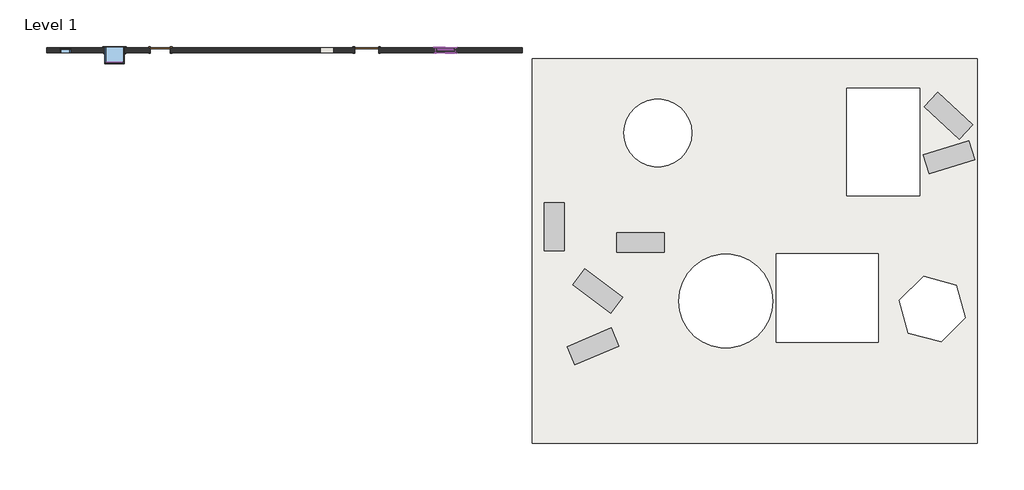
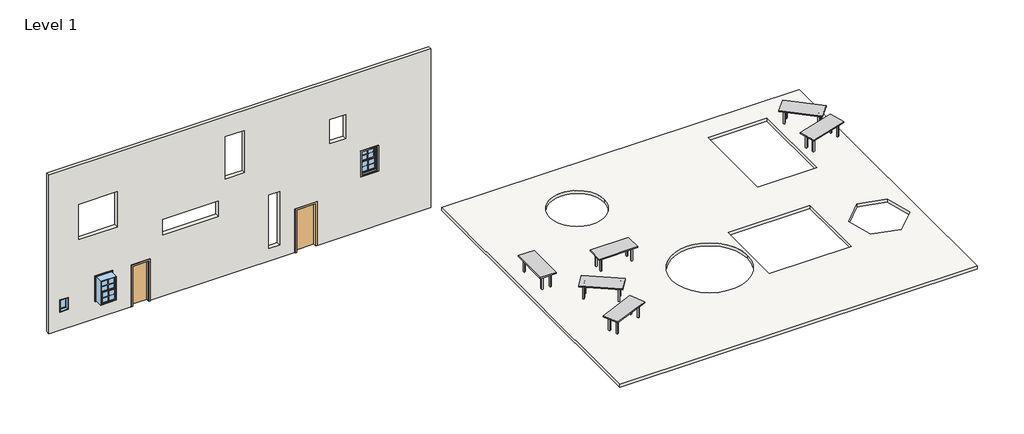
# One storey: 8 proxies, 6 furniture elements, 3 windows, 2 doors, 1 slab, 1 wall.
"""IFC4 building model written with IfcOpenShell, lengths in millimetres."""

import ifcopenshell
import ifcopenshell.guid

model = None  # the IFC model being written
_history = None  # IfcOwnerHistory: only IFC2X3 demands one
_inside = {}  # id of a spatial element -> (the spatial element, [elements in it])
_under = {}  # id of a project, library or spatial element -> (it, [spatial elements below it])
_declared = {}  # id of a project -> (the project, [libraries it declares])
_typed = {}  # id of a type object -> (the type object, [elements of that type])
_made_of = {}  # id of a material, layer set ... -> (it, [elements and type objects made of it])


def new_model(schema):
    """Start an empty IFC model of exactly this schema.

    Asked for "IFC4X3", IfcOpenShell would pick the latest addendum, in which some entities
    have other attributes; the version numbers below select the first issue.
    IFC2X3 requires an IfcOwnerHistory on every rooted entity: one is made here for all.
    """
    global model, _history
    if schema == "IFC4X3":
        model = ifcopenshell.file(schema_version=(4, 3, 0, 0))
    else:
        model = ifcopenshell.file(schema=schema)
    _inside.clear()
    _under.clear()
    _declared.clear()
    _typed.clear()
    _made_of.clear()
    _history = None
    if model.schema == "IFC2X3":
        org = make("IfcOrganization", Name="unknown")
        user = make(
            "IfcPersonAndOrganization",
            ThePerson=make("IfcPerson", FamilyName="unknown"),
            TheOrganization=org,
        )
        app = make(
            "IfcApplication",
            ApplicationDeveloper=org,
            Version="unknown",
            ApplicationFullName="unknown",
            ApplicationIdentifier="unknown",
        )
        _history = make(
            "IfcOwnerHistory",
            OwningUser=user,
            OwningApplication=app,
            ChangeAction="ADDED",
            CreationDate=0,
        )
    return model


def make(cls, **values):
    """One entity of the class cls with the attributes given. An attribute that is None is left unset."""
    return model.create_entity(
        cls, **{name: value for name, value in values.items() if value is not None}
    )


def rooted(cls, **values):
    """An entity with a GlobalId (a new one), such as an element, a storey or a relation."""
    return make(cls, GlobalId=ifcopenshell.guid.new(), OwnerHistory=_history, **values)


def si_unit(unit_type, name, prefix=None):
    """IfcSIUnit, for example si_unit("LENGTHUNIT", "METRE", prefix="MILLI")."""
    return make("IfcSIUnit", UnitType=unit_type, Prefix=prefix, Name=name)


def assignment(units):
    """IfcUnitAssignment: the units of a project."""
    return None if units is None else make("IfcUnitAssignment", Units=units)


def point(xyz):
    """IfcCartesianPoint."""
    return None if xyz is None else make("IfcCartesianPoint", Coordinates=xyz)


def direction(xyz):
    """IfcDirection."""
    return None if xyz is None else make("IfcDirection", DirectionRatios=xyz)


def frame(location, z_axis=None, x_axis=None):
    """IfcAxis2Placement3D, a coordinate frame: its origin and axes. An axis left out is left unset."""
    return make(
        "IfcAxis2Placement3D",
        Location=point(location),
        Axis=direction(z_axis),
        RefDirection=direction(x_axis),
    )


def frame_2d(location, x_axis=None):
    """IfcAxis2Placement2D, a coordinate frame in the plane: its origin and x axis."""
    return make(
        "IfcAxis2Placement2D", Location=point(location), RefDirection=direction(x_axis)
    )


def origin():
    """The frame at (0, 0, 0) with its axes left unset."""
    return frame((0.0, 0.0, 0.0))


def origin_with_axes():
    """The frame at (0, 0, 0) with the z axis (0, 0, 1) and the x axis (1, 0, 0) written out."""
    return frame((0.0, 0.0, 0.0), z_axis=(0.0, 0.0, 1.0), x_axis=(1.0, 0.0, 0.0))


def place(relative_to, where):
    """IfcLocalPlacement: puts the frame where relative to a parent placement (None: the world)."""
    return make(
        "IfcLocalPlacement", PlacementRelTo=relative_to, RelativePlacement=where
    )


def context(
    kind, dimensions, precision=None, world=None, true_north=None, identifier=None
):
    """IfcGeometricRepresentationContext, for example the 3D "Model" context."""
    return make(
        "IfcGeometricRepresentationContext",
        ContextIdentifier=identifier,
        ContextType=kind,
        CoordinateSpaceDimension=dimensions,
        Precision=precision,
        WorldCoordinateSystem=world,
        TrueNorth=true_north,
    )


def project(units=None, contexts=None):
    """IfcProject with its units and contexts."""
    return rooted(
        "IfcProject",
        Name="project",
        RepresentationContexts=contexts,
        UnitsInContext=assignment(units),
    )


def spatial(cls, under=None, at=None, **own):
    """A site, building, storey or space (cls), placed at a placement, below another one or the project."""
    s = rooted(cls, ObjectPlacement=at, **own)
    if under is not None:
        _under.setdefault(under.id(), (under, []))[1].append(s)
    return s


def polyline(points):
    """IfcPolyline through the points."""
    return make("IfcPolyline", Points=[point(p) for p in points])


def circle_curve(where, radius):
    """IfcCircle in the frame where."""
    return make("IfcCircle", Position=where, Radius=radius)


def trimmed(basis, trim1, trim2, sense, master):
    """IfcTrimmedCurve: the piece of a basis curve between two trims."""
    return make(
        "IfcTrimmedCurve",
        BasisCurve=basis,
        Trim1=trim1,
        Trim2=trim2,
        SenseAgreement=sense,
        MasterRepresentation=master,
    )


def segment(curve, same_sense, transition):
    """IfcCompositeCurveSegment."""
    return make(
        "IfcCompositeCurveSegment",
        Transition=transition,
        SameSense=same_sense,
        ParentCurve=curve,
    )


def composite_curve(segments, self_intersect=None):
    """IfcCompositeCurve: segments joined end to end."""
    return make("IfcCompositeCurve", Segments=segments, SelfIntersect=self_intersect)


def outline(outer, holes=None, kind="AREA"):
    """IfcArbitraryClosedProfileDef: a profile drawn as a closed curve; with holes, ...WithVoids."""
    if holes is None:
        return make("IfcArbitraryClosedProfileDef", ProfileType=kind, OuterCurve=outer)
    return make(
        "IfcArbitraryProfileDefWithVoids",
        ProfileType=kind,
        OuterCurve=outer,
        InnerCurves=holes,
    )


def extrude(swept, where, along, depth):
    """IfcExtrudedAreaSolid: the profile swept, set in the frame where, extruded along a direction by depth."""
    return make(
        "IfcExtrudedAreaSolid",
        SweptArea=swept,
        Position=where,
        ExtrudedDirection=direction(along),
        Depth=depth,
    )


def shape(context_of_items, identifier, shape_type, items):
    """IfcShapeRepresentation: the items that make up one representation, for example the "Body"."""
    return make(
        "IfcShapeRepresentation",
        ContextOfItems=context_of_items,
        RepresentationIdentifier=identifier,
        RepresentationType=shape_type,
        Items=items,
    )


def source(mapping_origin, context_of_items, identifier, shape_type, items):
    """IfcRepresentationMap: a shape defined once, which mapped items show again and again."""
    return make(
        "IfcRepresentationMap",
        MappingOrigin=mapping_origin,
        MappedRepresentation=shape(context_of_items, identifier, shape_type, items),
    )


def transform(
    local_origin,
    x_axis=None,
    y_axis=None,
    z_axis=None,
    scale=None,
    scale2=None,
    scale3=None,
    uniform=True,
):
    """IfcCartesianTransformationOperator3D, or its non-uniform kind. x_axis, y_axis, z_axis: its Axis1, 2, 3."""
    if uniform:
        return make(
            "IfcCartesianTransformationOperator3D",
            Axis1=direction(x_axis),
            Axis2=direction(y_axis),
            LocalOrigin=point(local_origin),
            Scale=scale,
            Axis3=direction(z_axis),
        )
    return make(
        "IfcCartesianTransformationOperator3DnonUniform",
        Axis1=direction(x_axis),
        Axis2=direction(y_axis),
        LocalOrigin=point(local_origin),
        Scale=scale,
        Axis3=direction(z_axis),
        Scale2=scale2,
        Scale3=scale3,
    )


def mapped(mapping_source, mapping_target):
    """IfcMappedItem: shows the shape of a source again, moved by a transform."""
    return make(
        "IfcMappedItem", MappingSource=mapping_source, MappingTarget=mapping_target
    )


def made_of(thing, what):
    """Note that an element or type object is made of a material, layer set ...; save() writes the relation."""
    if what is not None:
        _made_of.setdefault(what.id(), (what, []))[1].append(thing)
    return thing


def element(
    cls,
    number,
    at=None,
    inside=None,
    cuts=None,
    type_object=None,
    material=None,
    context=None,
    identifier="Body",
    shape_type=None,
    held_by="IfcProductDefinitionShape",
    body=None,
    shapes=None,
    **own,
):
    """One element of the class cls, such as IfcWall. Its Tag is "e" and its number.

    at: its placement. inside: the storey or other place that contains it. cuts: it is an
    opening in that element (IfcRelVoidsElement). A single representation is given by context,
    identifier, shape_type and body (its items); several are given by shapes. held_by: the class
    of the entity that holds the representations. save() writes the other relations.
    """
    e = rooted(cls, Tag="e%d" % number, ObjectPlacement=at, **own)
    if body is not None:
        shapes = [shape(context, identifier, shape_type, body)]
    if shapes is not None:
        e.Representation = make(held_by, Representations=shapes)
    if inside is not None:
        _inside.setdefault(inside.id(), (inside, []))[1].append(e)
    if cuts is not None:
        rooted(
            "IfcRelVoidsElement", RelatingBuildingElement=cuts, RelatedOpeningElement=e
        )
    if type_object is not None:
        _typed.setdefault(type_object.id(), (type_object, []))[1].append(e)
    return made_of(e, material)


def aggregate(whole, parts):
    """IfcRelAggregates: a whole, such as a stair, and the parts it consists of."""
    return rooted("IfcRelAggregates", RelatingObject=whole, RelatedObjects=parts)


def save(model, path):
    """Write the relations noted so far, then the file.

    IfcRelAggregates (storeys below a building ...), IfcRelContainedInSpatialStructure (elements
    in a storey), IfcRelDefinesByType, IfcRelAssociatesMaterial and IfcRelDeclares: one each for
    every whole, place, type object, material and project.
    """
    for whole, parts in _under.values():
        aggregate(whole, parts)
    for where, things in _inside.values():
        rooted(
            "IfcRelContainedInSpatialStructure",
            RelatedElements=things,
            RelatingStructure=where,
        )
    for kind, things in _typed.values():
        rooted("IfcRelDefinesByType", RelatedObjects=things, RelatingType=kind)
    for what, things in _made_of.values():
        rooted("IfcRelAssociatesMaterial", RelatedObjects=things, RelatingMaterial=what)
    for by, libraries in _declared.values():
        rooted("IfcRelDeclares", RelatingContext=by, RelatedDefinitions=libraries)
    model.write(path)


def m_muntin_pattern_2x2_m_muntin_pattern_2x2_aaec3afb(model_context):
    return source(origin(), model_context, "Body", "SweptSolid", [
        extrude(outline(polyline([(257.1375, -6.35), (257.1375, -298.8), (244.4375, -298.8), (244.4375, -6.35), (0.0, -6.35), (0.0, 6.35), (244.4375, 6.35), (244.4375, 298.8), (257.1375, 298.8), (257.1375, 6.35), (501.575, 6.35), (501.575, -6.35), (257.1375, -6.35)])), frame((0.0, 9.525, 0.0), z_axis=(0.0, 1.0, 0.0), x_axis=(0.0, 0.0, 1.0)), (0.0, 0.0, 1.0), 12.7),
        extrude(outline(polyline([(257.1375, -6.35), (257.1375, -298.8), (244.4375, -298.8), (244.4375, -6.35), (0.0, -6.35), (0.0, 6.35), (244.4375, 6.35), (244.4375, 298.8), (257.1375, 298.8), (257.1375, 6.35), (501.575, 6.35), (501.575, -6.35), (257.1375, -6.35)])), frame((0.0, -22.225, 0.0), z_axis=(0.0, 1.0, 0.0), x_axis=(0.0, 0.0, 1.0)), (0.0, 0.0, 1.0), 12.7),
    ])


def m_trim_window_exterior_flat_with_sill_e7ff6350(model_context):
    return source(origin(), model_context, "Body", "SweptSolid", [
        extrude(outline(polyline([(435.0, -1220.4323709), (435.0, -1280.4323709), (-435.0, -1280.4323709), (-435.0, -1220.4323709), (435.0, -1220.4323709)])), origin_with_axes(), (0.0, 0.0, 1.0), 19.05),
        extrude(outline(polyline([(-1230.0, 38.1), (-1202.4580645, 38.1), (-1200.0, 19.05), (-1200.0, 0.0), (-1220.4323709, 0.0), (-1220.4323709, 19.05), (-1230.0, 19.05), (-1230.0, 38.1)])), frame((-447.7, 0.0, 0.0), z_axis=(1.0, 0.0, 0.0), x_axis=(0.0, 1.0, 0.0)), (0.0, 0.0, 1.0), 895.4),
        extrude(outline(polyline([(-435.0, 60.0), (435.0, 60.0), (435.0, -1200.0), (375.0, -1200.0), (375.0, 0.0), (-375.0, 0.0), (-375.0, -1200.0), (-435.0, -1200.0), (-435.0, 60.0)])), origin_with_axes(), (0.0, 0.0, 1.0), 19.05),
    ])


def m_trim_window_interior_flat_picture_frame_31bd2320(model_context):
    return source(origin(), model_context, "Body", "SweptSolid", [
        extrude(outline(polyline([(422.3, 47.3), (422.3, -1247.3), (-422.3, -1247.3), (-422.3, 47.3), (422.3, 47.3)]), holes=[polyline([(362.3, -12.7), (-362.3, -12.7), (-362.3, -1187.3), (362.3, -1187.3), (362.3, -12.7)])]), origin_with_axes(), (0.0, 0.0, 1.0), 30.0),
    ])


def m_single_flush_0762_x_2032mm_0c256fab(model_context):
    return source(origin(), model_context, "Body", "SweptSolid", [
        extrude(outline(polyline([(2108.0, -457.0), (0.0, -457.0), (0.0, -381.0), (2032.0, -381.0), (2032.0, 381.0), (0.0, 381.0), (0.0, 457.0), (2108.0, 457.0), (2108.0, -457.0)])), frame((0.0, 100.0, 0.0), z_axis=(0.0, 1.0, 0.0), x_axis=(0.0, 0.0, 1.0)), (0.0, 0.0, 1.0), 25.0),
        extrude(outline(polyline([(2108.0, 457.0), (2108.0, -457.0), (0.0, -457.0), (0.0, -381.0), (2032.0, -381.0), (2032.0, 381.0), (0.0, 381.0), (0.0, 457.0), (2108.0, 457.0)])), frame((0.0, -125.0, 0.0), z_axis=(0.0, 1.0, 0.0), x_axis=(0.0, 0.0, 1.0)), (0.0, 0.0, 1.0), 25.0),
        extrude(outline(polyline([(381.0, 49.0), (-381.0, 49.0), (-381.0, 100.0), (381.0, 100.0), (381.0, 49.0)])), origin_with_axes(), (0.0, 0.0, 1.0), 2032.0),
    ])


def m_single_flush_0915_x_2134mm_727434cd(model_context):
    return source(origin(), model_context, "Body", "SweptSolid", [
        extrude(outline(polyline([(2210.0, -533.5), (0.0, -533.5), (0.0, -457.5), (2134.0, -457.5), (2134.0, 457.5), (0.0, 457.5), (0.0, 533.5), (2210.0, 533.5), (2210.0, -533.5)])), frame((0.0, -125.0, 0.0), z_axis=(0.0, 1.0, 0.0), x_axis=(0.0, 0.0, 1.0)), (0.0, 0.0, 1.0), 25.0),
        extrude(outline(polyline([(2210.0, 533.5), (2210.0, -533.5), (0.0, -533.5), (0.0, -457.5), (2134.0, -457.5), (2134.0, 457.5), (0.0, 457.5), (0.0, 533.5), (2210.0, 533.5)])), frame((0.0, 100.0, 0.0), z_axis=(0.0, 1.0, 0.0), x_axis=(0.0, 0.0, 1.0)), (0.0, 0.0, 1.0), 25.0),
        extrude(outline(polyline([(457.5, -49.0), (457.5, -100.0), (-457.5, -100.0), (-457.5, -49.0), (457.5, -49.0)])), origin_with_axes(), (0.0, 0.0, 1.0), 2134.0),
    ])


def m_table_rectangular_1830_x_0762mm_a0b3b7a0(model_context):
    return source(origin(), model_context, "Body", "SweptSolid", [
        extrude(outline(polyline([(699.1, 190.5), (699.1, 165.1), (-699.1, 165.1), (-699.1, 190.5), (699.1, 190.5)])), frame((0.0, 0.0, 609.6), z_axis=(0.0, 0.0, 1.0), x_axis=(1.0, 0.0, 0.0)), (0.0, 0.0, 1.0), 101.6),
        extrude(outline(polyline([(699.1, -190.5), (-699.1, -190.5), (-699.1, -165.1), (699.1, -165.1), (699.1, -190.5)])), frame((0.0, 0.0, 609.6), z_axis=(0.0, 0.0, 1.0), x_axis=(1.0, 0.0, 0.0)), (0.0, 0.0, 1.0), 101.6),
        extrude(outline(polyline([(-711.8, -165.1), (-737.2, -165.1), (-737.2, 165.1), (-711.8, 165.1), (-711.8, -165.1)])), frame((0.0, 0.0, 609.6), z_axis=(0.0, 0.0, 1.0), x_axis=(1.0, 0.0, 0.0)), (0.0, 0.0, 1.0), 101.6),
        extrude(outline(polyline([(711.8, -165.1), (711.8, 165.1), (737.2, 165.1), (737.2, -165.1), (711.8, -165.1)])), frame((0.0, 0.0, 609.6), z_axis=(0.0, 0.0, 1.0), x_axis=(1.0, 0.0, 0.0)), (0.0, 0.0, 1.0), 101.6),
        extrude(outline(polyline([(915.0, 381.0), (915.0, -381.0), (-915.0, -381.0), (-915.0, 381.0), (915.0, 381.0)])), frame((0.0, 0.0, 711.2), z_axis=(0.0, 0.0, 1.0), x_axis=(1.0, 0.0, 0.0)), (0.0, 0.0, 1.0), 50.8),
        extrude(outline(polyline([(-699.1, 228.6), (-699.1, 165.1), (-762.6, 165.1), (-762.6, 228.6), (-699.1, 228.6)])), origin_with_axes(), (0.0, 0.0, 1.0), 711.2),
        extrude(outline(polyline([(699.1, 228.6), (762.6, 228.6), (762.6, 165.1), (699.1, 165.1), (699.1, 228.6)])), origin_with_axes(), (0.0, 0.0, 1.0), 711.2),
        extrude(outline(polyline([(-699.1, -228.6), (-762.6, -228.6), (-762.6, -165.1), (-699.1, -165.1), (-699.1, -228.6)])), origin_with_axes(), (0.0, 0.0, 1.0), 711.2),
        extrude(outline(polyline([(699.1, -228.6), (699.1, -165.1), (762.6, -165.1), (762.6, -228.6), (699.1, -228.6)])), origin_with_axes(), (0.0, 0.0, 1.0), 711.2),
    ])


def m_table_rectangular_1830_x_0762mm_ec068ed4(model_context):
    return source(origin(), model_context, "Body", "SweptSolid", [
        extrude(outline(polyline([(699.1, -190.5), (-699.1, -190.5), (-699.1, -165.1), (699.1, -165.1), (699.1, -190.5)])), frame((0.0, 0.0, 609.6), z_axis=(0.0, 0.0, 1.0), x_axis=(1.0, 0.0, 0.0)), (0.0, 0.0, 1.0), 101.6),
        extrude(outline(polyline([(699.1, 190.5), (699.1, 165.1), (-699.1, 165.1), (-699.1, 190.5), (699.1, 190.5)])), frame((0.0, 0.0, 609.6), z_axis=(0.0, 0.0, 1.0), x_axis=(1.0, 0.0, 0.0)), (0.0, 0.0, 1.0), 101.6),
        extrude(outline(polyline([(-711.8, 165.1), (-711.8, -165.1), (-737.2, -165.1), (-737.2, 165.1), (-711.8, 165.1)])), frame((0.0, 0.0, 609.6), z_axis=(0.0, 0.0, 1.0), x_axis=(1.0, 0.0, 0.0)), (0.0, 0.0, 1.0), 101.6),
        extrude(outline(polyline([(711.8, 165.1), (737.2, 165.1), (737.2, -165.1), (711.8, -165.1), (711.8, 165.1)])), frame((0.0, 0.0, 609.6), z_axis=(0.0, 0.0, 1.0), x_axis=(1.0, 0.0, 0.0)), (0.0, 0.0, 1.0), 101.6),
        extrude(outline(polyline([(915.0, -381.0), (-915.0, -381.0), (-915.0, 381.0), (915.0, 381.0), (915.0, -381.0)])), frame((0.0, 0.0, 711.2), z_axis=(0.0, 0.0, 1.0), x_axis=(1.0, 0.0, 0.0)), (0.0, 0.0, 1.0), 50.8),
        extrude(outline(polyline([(-699.1, -228.6), (-762.6, -228.6), (-762.6, -165.1), (-699.1, -165.1), (-699.1, -228.6)])), origin_with_axes(), (0.0, 0.0, 1.0), 711.2),
        extrude(outline(polyline([(699.1, -228.6), (699.1, -165.1), (762.6, -165.1), (762.6, -228.6), (699.1, -228.6)])), origin_with_axes(), (0.0, 0.0, 1.0), 711.2),
        extrude(outline(polyline([(-699.1, 228.6), (-699.1, 165.1), (-762.6, 165.1), (-762.6, 228.6), (-699.1, 228.6)])), origin_with_axes(), (0.0, 0.0, 1.0), 711.2),
        extrude(outline(polyline([(699.1, 228.6), (762.6, 228.6), (762.6, 165.1), (699.1, 165.1), (699.1, 228.6)])), origin_with_axes(), (0.0, 0.0, 1.0), 711.2),
    ])


def m_fixed_0406_x_0610mm_8205b201(model_context):
    return source(origin(), model_context, "Body", "SweptSolid", [
        extrude(outline(polyline([(-140.0, 78.0), (140.0, 78.0), (140.0, 66.0), (-140.0, 66.0), (-140.0, 78.0)])), frame((0.0, 0.0, 978.0), z_axis=(0.0, 0.0, 1.0), x_axis=(1.0, 0.0, 0.0)), (0.0, 0.0, 1.0), 484.0),
        extrude(outline(polyline([(1506.0, -184.0), (934.0, -184.0), (934.0, 184.0), (1506.0, 184.0), (1506.0, -184.0)]), holes=[polyline([(1462.0, -140.0), (1462.0, 140.0), (978.0, 140.0), (978.0, -140.0), (1462.0, -140.0)])]), frame((0.0, 50.0, 0.0), z_axis=(0.0, 1.0, 0.0), x_axis=(0.0, 0.0, 1.0)), (0.0, 0.0, 1.0), 44.0),
        extrude(outline(polyline([(1525.0, -203.0), (915.0, -203.0), (915.0, 203.0), (1525.0, 203.0), (1525.0, -203.0)]), holes=[polyline([(1506.0, -184.0), (1506.0, 184.0), (934.0, 184.0), (934.0, -184.0), (1506.0, -184.0)])]), frame((0.0, 50.0, 0.0), z_axis=(0.0, 1.0, 0.0), x_axis=(0.0, 0.0, 1.0)), (0.0, 0.0, 1.0), 63.0),
        extrude(outline(polyline([(1525.0, -203.0), (915.0, -203.0), (915.0, 203.0), (1525.0, 203.0), (1525.0, -203.0)]), holes=[polyline([(1493.0, -171.0), (1493.0, 171.0), (947.0, 171.0), (947.0, -171.0), (1493.0, -171.0)])]), frame((0.0, -87.0, 0.0), z_axis=(0.0, 1.0, 0.0), x_axis=(0.0, 0.0, 1.0)), (0.0, 0.0, 1.0), 137.0),
    ])


def m_window_double_hung_750_x_1200mm_e21ea802(model_context):
    return source(origin(), model_context, "Body", "SweptSolid", [
        extrude(outline(polyline([(298.8, -469.85), (298.8, -476.2), (-298.8, -476.2), (-298.8, -469.85), (298.8, -469.85)])), frame((0.0, 0.0, 990.6), z_axis=(0.0, 0.0, 1.0), x_axis=(1.0, 0.0, 0.0)), (0.0, 0.0, 1.0), 501.575),
        extrude(outline(polyline([(-298.8, -482.55), (298.8, -482.55), (298.8, -488.9), (-298.8, -488.9), (-298.8, -482.55)])), frame((0.0, 0.0, 990.6), z_axis=(0.0, 0.0, 1.0), x_axis=(1.0, 0.0, 0.0)), (0.0, 0.0, 1.0), 501.575),
        extrude(outline(polyline([(298.8, -425.4), (298.8, -431.75), (-298.8, -431.75), (-298.8, -425.4), (298.8, -425.4)])), frame((0.0, 0.0, 1536.625), z_axis=(0.0, 0.0, 1.0), x_axis=(1.0, 0.0, 0.0)), (0.0, 0.0, 1.0), 501.575),
        extrude(outline(polyline([(-298.8, -438.1), (298.8, -438.1), (298.8, -444.45), (-298.8, -444.45), (-298.8, -438.1)])), frame((0.0, 0.0, 1536.625), z_axis=(0.0, 0.0, 1.0), x_axis=(1.0, 0.0, 0.0)), (0.0, 0.0, 1.0), 501.575),
        extrude(outline(polyline([(1536.625, -343.25), (946.15, -343.25), (946.15, 343.25), (1536.625, 343.25), (1536.625, -343.25)]), holes=[polyline([(1492.175, 298.8), (990.6, 298.8), (990.6, -298.8), (1492.175, -298.8), (1492.175, 298.8)])]), frame((0.0, -501.6, 0.0), z_axis=(0.0, 1.0, 0.0), x_axis=(0.0, 0.0, 1.0)), (0.0, 0.0, 1.0), 44.45),
        extrude(outline(polyline([(2082.65, -343.25), (1492.175, -343.25), (1492.175, 343.25), (2082.65, 343.25), (2082.65, -343.25)]), holes=[polyline([(2038.2, 298.8), (1536.625, 298.8), (1536.625, -298.8), (2038.2, -298.8), (2038.2, 298.8)])]), frame((0.0, -457.15, 0.0), z_axis=(0.0, 1.0, 0.0), x_axis=(0.0, 0.0, 1.0)), (0.0, 0.0, 1.0), 44.45),
        extrude(outline(polyline([(2114.4, -375.0), (914.4, -375.0), (914.4, 375.0), (2114.4, 375.0), (2114.4, -375.0)]), holes=[polyline([(2082.65, 343.25), (946.15, 343.25), (946.15, -343.25), (2082.65, -343.25), (2082.65, 343.25)])]), frame((0.0, -514.3, 0.0), z_axis=(0.0, 1.0, 0.0), x_axis=(0.0, 0.0, 1.0)), (0.0, 0.0, 1.0), 633.35),
    ])


def m_window_double_hung_750_x_1200mm_41070976(model_context):
    return source(origin(), model_context, "Body", "SweptSolid", [
        extrude(outline(polyline([(298.8, 30.15), (298.8, 23.8), (-298.8, 23.8), (-298.8, 30.15), (298.8, 30.15)])), frame((0.0, 0.0, 990.6), z_axis=(0.0, 0.0, 1.0), x_axis=(1.0, 0.0, 0.0)), (0.0, 0.0, 1.0), 501.575),
        extrude(outline(polyline([(-298.8, 17.45), (298.8, 17.45), (298.8, 11.1), (-298.8, 11.1), (-298.8, 17.45)])), frame((0.0, 0.0, 990.6), z_axis=(0.0, 0.0, 1.0), x_axis=(1.0, 0.0, 0.0)), (0.0, 0.0, 1.0), 501.575),
        extrude(outline(polyline([(298.8, 74.6), (298.8, 68.25), (-298.8, 68.25), (-298.8, 74.6), (298.8, 74.6)])), frame((0.0, 0.0, 1536.625), z_axis=(0.0, 0.0, 1.0), x_axis=(1.0, 0.0, 0.0)), (0.0, 0.0, 1.0), 501.575),
        extrude(outline(polyline([(-298.8, 61.9), (298.8, 61.9), (298.8, 55.55), (-298.8, 55.55), (-298.8, 61.9)])), frame((0.0, 0.0, 1536.625), z_axis=(0.0, 0.0, 1.0), x_axis=(1.0, 0.0, 0.0)), (0.0, 0.0, 1.0), 501.575),
        extrude(outline(polyline([(1536.625, -343.25), (946.15, -343.25), (946.15, 343.25), (1536.625, 343.25), (1536.625, -343.25)]), holes=[polyline([(1492.175, 298.8), (990.6, 298.8), (990.6, -298.8), (1492.175, -298.8), (1492.175, 298.8)])]), frame((0.0, -1.6, 0.0), z_axis=(0.0, 1.0, 0.0), x_axis=(0.0, 0.0, 1.0)), (0.0, 0.0, 1.0), 44.45),
        extrude(outline(polyline([(2082.65, -343.25), (1492.175, -343.25), (1492.175, 343.25), (2082.65, 343.25), (2082.65, -343.25)]), holes=[polyline([(2038.2, 298.8), (1536.625, 298.8), (1536.625, -298.8), (2038.2, -298.8), (2038.2, 298.8)])]), frame((0.0, 42.85, 0.0), z_axis=(0.0, 1.0, 0.0), x_axis=(0.0, 0.0, 1.0)), (0.0, 0.0, 1.0), 44.45),
        extrude(outline(polyline([(2114.4, -375.0), (914.4, -375.0), (914.4, 375.0), (2114.4, 375.0), (2114.4, -375.0)]), holes=[polyline([(2082.65, 343.25), (946.15, 343.25), (946.15, -343.25), (2082.65, -343.25), (2082.65, 343.25)])]), frame((0.0, -14.3, 0.0), z_axis=(0.0, 1.0, 0.0), x_axis=(0.0, 0.0, 1.0)), (0.0, 0.0, 1.0), 133.35),
        extrude(outline(polyline([(2114.4, 375.0), (2114.4, -375.0), (914.4, -375.0), (914.4, 375.0), (2114.4, 375.0)]), holes=[polyline([(2095.35, 355.95), (933.45, 355.95), (933.45, -355.95), (2095.35, -355.95), (2095.35, 355.95)])]), frame((0.0, -100.0, 0.0), z_axis=(0.0, 1.0, 0.0), x_axis=(0.0, 0.0, 1.0)), (0.0, 0.0, 1.0), 85.7),
    ])


model = new_model("IFC4")

# Units and contexts
model_context = context("Model", 3, world=origin())
ifc_project = project(units=[si_unit("LENGTHUNIT", "METRE", prefix="MILLI")], contexts=[model_context])

# Site, building, storey
site = spatial("IfcSite", under=ifc_project)
building = spatial("IfcBuilding", under=site)
storey = spatial("IfcBuildingStorey", under=building, Name="Level 1", Elevation=0.0)

# Proxies
placement = place(None, origin())
m_muntin_pattern_2x2_m_muntin_pattern_2x2_shape = m_muntin_pattern_2x2_m_muntin_pattern_2x2_aaec3afb(model_context)
element("IfcBuildingElementProxy", 1, Name="M_Muntin Pattern_2x2 : M_Muntin Pattern_2x2", ObjectType="M_Muntin Pattern_2x2 : M_Muntin Pattern_2x2", at=placement, inside=storey, context=model_context, shape_type="MappedRepresentation", body=[
    mapped(m_muntin_pattern_2x2_m_muntin_pattern_2x2_shape, transform((-13755.2543844, 2099.5505832, 3404.9440493), x_axis=(1.0, 0.0, 0.0), y_axis=(0.0, 1.0, 0.0), z_axis=(0.0, 0.0, 1.0))),
])
element("IfcBuildingElementProxy", 2, Name="M_Muntin Pattern_2x2 : M_Muntin Pattern_2x2", ObjectType="M_Muntin Pattern_2x2 : M_Muntin Pattern_2x2", at=placement, inside=storey, context=model_context, shape_type="MappedRepresentation", body=[
    mapped(m_muntin_pattern_2x2_m_muntin_pattern_2x2_shape, transform((-13755.2543844, 2055.1005832, 2858.9190493), x_axis=(1.0, 0.0, 0.0), y_axis=(0.0, 1.0, 0.0), z_axis=(0.0, 0.0, 1.0))),
])
element("IfcBuildingElementProxy", 3, Name="M_Muntin Pattern_2x2 : M_Muntin Pattern_2x2", ObjectType="M_Muntin Pattern_2x2 : M_Muntin Pattern_2x2", at=placement, inside=storey, context=model_context, shape_type="MappedRepresentation", body=[
    mapped(m_muntin_pattern_2x2_m_muntin_pattern_2x2_shape, transform((-26415.5284847, 1599.5505832, 1536.625), x_axis=(1.0, 0.0, 0.0), y_axis=(0.0, 1.0, 0.0), z_axis=(0.0, 0.0, 1.0))),
])
element("IfcBuildingElementProxy", 4, Name="M_Muntin Pattern_2x2 : M_Muntin Pattern_2x2", ObjectType="M_Muntin Pattern_2x2 : M_Muntin Pattern_2x2", at=placement, inside=storey, context=model_context, shape_type="MappedRepresentation", body=[
    mapped(m_muntin_pattern_2x2_m_muntin_pattern_2x2_shape, transform((-26415.5284847, 1555.1005832, 990.6), x_axis=(1.0, 0.0, 0.0), y_axis=(0.0, 1.0, 0.0), z_axis=(0.0, 0.0, 1.0))),
])
m_trim_window_exterior_flat_with_sill_shape = m_trim_window_exterior_flat_with_sill_e7ff6350(model_context)
element("IfcBuildingElementProxy", 5, Name="M_Trim-Window-Exterior-Flat : with Sill", ObjectType="M_Trim-Window-Exterior-Flat : with Sill", at=placement, inside=storey, context=model_context, shape_type="MappedRepresentation", body=[
    mapped(m_trim_window_exterior_flat_with_sill_shape, transform((-13755.2543844, 2134.4755832, 3982.7190493), x_axis=(-1.0, 0.0, 0.0), y_axis=(0.0, 0.0, 1.0), z_axis=(0.0, 1.0, 0.0))),
])
element("IfcBuildingElementProxy", 6, Name="M_Trim-Window-Exterior-Flat : with Sill", ObjectType="M_Trim-Window-Exterior-Flat : with Sill", at=placement, inside=storey, context=model_context, shape_type="MappedRepresentation", body=[
    mapped(m_trim_window_exterior_flat_with_sill_shape, transform((-26415.5284847, 2134.4755832, 2114.4), x_axis=(-1.0, 0.0, 0.0), y_axis=(0.0, 0.0, 1.0), z_axis=(0.0, 1.0, 0.0))),
])
m_trim_window_interior_flat_picture_frame_shape = m_trim_window_interior_flat_picture_frame_31bd2320(model_context)
element("IfcBuildingElementProxy", 7, Name="M_Trim-Window-Interior-Flat : Picture Frame", ObjectType="M_Trim-Window-Interior-Flat : Picture Frame", at=placement, inside=storey, context=model_context, shape_type="MappedRepresentation", body=[
    mapped(m_trim_window_interior_flat_picture_frame_shape, transform((-13755.2543844, 1934.4755832, 3982.7190493), x_axis=(1.0, 0.0, 0.0), y_axis=(0.0, 0.0, 1.0), z_axis=(0.0, -1.0, 0.0))),
])
element("IfcBuildingElementProxy", 8, Name="M_Trim-Window-Interior-Flat : Picture Frame", ObjectType="M_Trim-Window-Interior-Flat : Picture Frame", at=placement, inside=storey, context=model_context, shape_type="MappedRepresentation", body=[
    mapped(m_trim_window_interior_flat_picture_frame_shape, transform((-26415.5284847, 1934.4755832, 2114.4), x_axis=(1.0, 0.0, 0.0), y_axis=(0.0, 0.0, 1.0), z_axis=(0.0, -1.0, 0.0))),
])

# Doors
m_single_flush_0762_x_2032mm_shape = m_single_flush_0762_x_2032mm_0c256fab(model_context)
element("IfcDoor", 9, ObjectType="M_Single-Flush : 0762 x 2032mm", at=placement, inside=storey, context=model_context, shape_type="MappedRepresentation", body=[
    mapped(m_single_flush_0762_x_2032mm_shape, transform((-24659.5284847, 2034.4755832, 0.0), x_axis=(1.0, 0.0, 0.0), y_axis=(0.0, 1.0, 0.0), z_axis=(0.0, 0.0, 1.0))),
])
m_single_flush_0915_x_2134mm_shape = m_single_flush_0915_x_2134mm_727434cd(model_context)
element("IfcDoor", 10, ObjectType="M_Single-Flush : 0915 x 2134mm", at=placement, inside=storey, context=model_context, shape_type="MappedRepresentation", body=[
    mapped(m_single_flush_0915_x_2134mm_shape, transform((-16774.8897659, 2034.4755832, 0.0), x_axis=(-1.0, 0.0, 0.0), y_axis=(0.0, -1.0, 0.0), z_axis=(0.0, 0.0, 1.0))),
])

# Furniture
m_table_rectangular_1830_x_0762mm_shape = m_table_rectangular_1830_x_0762mm_a0b3b7a0(model_context)
element("IfcFurniture", 11, ObjectType="M_Table-Rectangular : 1830 x 0762mm", at=placement, inside=storey, context=model_context, shape_type="MappedRepresentation", body=[
    mapped(m_table_rectangular_1830_x_0762mm_shape, transform((-6296.1972949, -5323.9774044, 0.0), x_axis=(-1.0, 0.0, 0.0), y_axis=(0.0, -1.0, 0.0), z_axis=(0.0, 0.0, 1.0))),
])
element("IfcFurniture", 12, ObjectType="M_Table-Rectangular : 1830 x 0762mm", at=placement, inside=storey, context=model_context, shape_type="MappedRepresentation", body=[
    mapped(m_table_rectangular_1830_x_0762mm_shape, transform((-7934.3893105, -7176.9572862, 0.0), x_axis=(0.7986355100472892, -0.601815023152053, 0.0), y_axis=(0.601815023152053, 0.7986355100472892, 0.0), z_axis=(0.0, 0.0, 1.0))),
])
element("IfcFurniture", 13, ObjectType="M_Table-Rectangular : 1830 x 0762mm", at=placement, inside=storey, context=model_context, shape_type="MappedRepresentation", body=[
    mapped(m_table_rectangular_1830_x_0762mm_shape, transform((-9596.1972949, -4723.9774044, 0.0), x_axis=(0.0, 1.0, 0.0), y_axis=(-1.0, 0.0, 0.0), z_axis=(0.0, 0.0, 1.0))),
])
element("IfcFurniture", 14, ObjectType="M_Table-Rectangular : 1830 x 0762mm", at=placement, inside=storey, context=model_context, shape_type="MappedRepresentation", body=[
    mapped(m_table_rectangular_1830_x_0762mm_shape, transform((-8112.0141227, -9301.6688903, 0.0), x_axis=(0.9205048534524458, 0.39073112848926067, 0.0), y_axis=(-0.39073112848926067, 0.9205048534524458, 0.0), z_axis=(0.0, 0.0, 1.0))),
])
m_table_rectangular_1830_x_0762mm_2_shape = m_table_rectangular_1830_x_0762mm_ec068ed4(model_context)
element("IfcFurniture", 15, ObjectType="M_Table-Rectangular : 1830 x 0762mm", at=placement, inside=storey, context=model_context, shape_type="MappedRepresentation", body=[
    mapped(m_table_rectangular_1830_x_0762mm_2_shape, transform((5509.5543182, -2054.6922097, 0.0), x_axis=(-0.9563047559630324, -0.2923717047227468, 0.0), y_axis=(0.2923717047227468, -0.9563047559630324, 0.0), z_axis=(0.0, 0.0, 1.0))),
])
element("IfcFurniture", 16, ObjectType="M_Table-Rectangular : 1830 x 0762mm", at=placement, inside=storey, context=model_context, shape_type="MappedRepresentation", body=[
    mapped(m_table_rectangular_1830_x_0762mm_2_shape, transform((5492.8202713, -469.7512134, 0.0), x_axis=(-0.7313537016191695, 0.6819983600624996, 0.0), y_axis=(-0.6819983600624996, -0.7313537016191695, 0.0), z_axis=(0.0, 0.0, 1.0))),
])

# Slab
element("IfcSlab", 17, ObjectType="Generic 150mm", at=placement, inside=storey, context=model_context, shape_type="SweptSolid", body=[
    extrude(outline(polyline([(-10438.0920872, 1704.9536342), (6597.1361468, 1704.9536342), (6597.1361468, -12995.0463658), (-10438.0920872, -12995.0463658), (-10438.0920872, 1704.9536342)]), holes=[polyline([(-1096.2822975, -5745.5612839), (-1096.2822975, -9145.5612839), (2803.7177025, -9145.5612839), (2803.7177025, -5745.5612839), (-1096.2822975, -5745.5612839)]), composite_curve([segment(trimmed(circle_curve(frame_2d((-3026.5132944, -7566.8871411)), 1800.0), [point((-1226.5132944, -7566.8871411))], [point((-4826.5132944, -7566.8871411))], True, "CARTESIAN"), True, "CONTINUOUS"), segment(trimmed(circle_curve(frame_2d((-3026.5132944, -7566.8871411)), 1800.0), [point((-4826.5132944, -7566.8871411))], [point((-1226.5132944, -7566.8871411))], True, "CARTESIAN"), True, "CONTINUOUS")], self_intersect=False), polyline([(3950.2905395, -8793.2666419), (5205.9941136, -9129.7314005), (6125.2329292, -8210.492585), (5788.7681706, -6954.7890108), (4533.0645964, -6618.3242522), (3613.8257808, -7537.5630677), (3950.2905395, -8793.2666419)]), polyline([(4397.1361468, 574.3329665), (1597.1361468, 574.3329665), (1597.1361468, -3525.6670335), (4397.1361468, -3525.6670335), (4397.1361468, 574.3329665)]), composite_curve([segment(trimmed(circle_curve(frame_2d((-5632.920233, -1133.8213408)), 1300.0), [point((-4332.920233, -1133.8213408))], [point((-6932.920233, -1133.8213408))], True, "CARTESIAN"), True, "CONTINUOUS"), segment(trimmed(circle_curve(frame_2d((-5632.920233, -1133.8213408)), 1300.0), [point((-6932.920233, -1133.8213408))], [point((-4332.920233, -1133.8213408))], True, "CARTESIAN"), True, "CONTINUOUS")], self_intersect=False)]), frame((0.0, 0.0, -150.0), z_axis=(0.0, 0.0, 1.0), x_axis=(1.0, 0.0, 0.0)), (0.0, 0.0, 1.0), 150.0),
])

# Wall
element("IfcWall", 18, ObjectType="Generic - 200mm", at=placement, inside=storey, context=model_context, shape_type="SweptSolid", body=[
    extrude(outline(polyline([(8000.0, -29017.3897659), (0.0, -29017.3897659), (0.0, -25040.5284847), (2032.0, -25040.5284847), (2032.0, -24278.5284847), (0.0, -24278.5284847), (0.0, -17232.3897659), (2134.0, -17232.3897659), (2134.0, -16317.3897659), (0.0, -16317.3897659), (0.0, -10817.3897659), (8000.0, -10817.3897659), (8000.0, -29017.3897659)]), holes=[polyline([(915.0, -28496.5284847), (1525.0, -28496.5284847), (1525.0, -28090.5284847), (915.0, -28090.5284847), (915.0, -28496.5284847)]), polyline([(914.4, -26790.5284847), (2114.4, -26790.5284847), (2114.4, -26040.5284847), (914.4, -26040.5284847), (914.4, -26790.5284847)]), polyline([(2782.7190493, -14130.2543844), (3982.7190493, -14130.2543844), (3982.7190493, -13380.2543844), (2782.7190493, -13380.2543844), (2782.7190493, -14130.2543844)]), polyline([(4914.4, -15639.9853759), (6114.4, -15639.9853759), (6114.4, -14889.9853759), (4914.4, -14889.9853759), (4914.4, -15639.9853759)]), polyline([(4866.0, -19702.3897659), (4866.0, -20617.3897659), (7000.0, -20617.3897659), (7000.0, -19702.3897659), (4866.0, -19702.3897659)]), polyline([(3328.9271244, -18544.8897659), (3328.9271244, -18024.3599995), (634.0, -18024.3599995), (634.0, -18544.8897659), (3328.9271244, -18544.8897659)]), polyline([(3873.453269, -23605.3752389), (3873.453269, -20944.8897659), (3100.0, -20944.8897659), (3100.0, -23605.3752389), (3873.453269, -23605.3752389)]), polyline([(6036.9886823, -27608.1535838), (6036.9886823, -25757.3810809), (4260.1064286, -25757.3810809), (4260.1064286, -27608.1535838), (6036.9886823, -27608.1535838)])]), frame((0.0, 1934.4755832, 0.0), z_axis=(0.0, 1.0, 0.0), x_axis=(0.0, 0.0, 1.0)), (0.0, 0.0, 1.0), 200.0),
])

# Windows
m_fixed_0406_x_0610mm_shape = m_fixed_0406_x_0610mm_8205b201(model_context)
element("IfcWindow", 19, ObjectType="M_Fixed : 0406 x 0610mm", at=placement, inside=storey, context=model_context, shape_type="MappedRepresentation", body=[
    mapped(m_fixed_0406_x_0610mm_shape, transform((-28293.5284847, 2021.4755832, 0.0), x_axis=(1.0, 0.0, 0.0), y_axis=(0.0, 1.0, 0.0), z_axis=(0.0, 0.0, 1.0))),
])
m_window_double_hung_750_x_1200mm_shape = m_window_double_hung_750_x_1200mm_e21ea802(model_context)
element("IfcWindow", 20, ObjectType="M_Window-Double-Hung : 750 x 1200mm", at=placement, inside=storey, context=model_context, shape_type="MappedRepresentation", body=[
    mapped(m_window_double_hung_750_x_1200mm_shape, transform((-26415.5284847, 2034.4755832, 0.0), x_axis=(1.0, 0.0, 0.0), y_axis=(0.0, 1.0, 0.0), z_axis=(0.0, 0.0, 1.0))),
])
m_window_double_hung_750_x_1200mm_2_shape = m_window_double_hung_750_x_1200mm_41070976(model_context)
element("IfcWindow", 21, ObjectType="M_Window-Double-Hung : 750 x 1200mm", at=placement, inside=storey, context=model_context, shape_type="MappedRepresentation", body=[
    mapped(m_window_double_hung_750_x_1200mm_2_shape, transform((-13755.2543844, 2034.4755832, 1868.3190493), x_axis=(1.0, 0.0, 0.0), y_axis=(0.0, 1.0, 0.0), z_axis=(0.0, 0.0, 1.0))),
])

save(model, "model.ifc")

# Revit data of these elements
# Project information
#   Project Issue Date = "Issue Date"
#   Project Status = "Project Status"
#   Client Name = "Owner"
#   Project Address = "Enter address here"
#   Project Name = "Project Name"
#   Project Number = "0001"
# Type "M_Muntin Pattern_2x2 : M_Muntin Pattern_2x2"
#   Width [instance default] = 1200 mm
#   Thickness = 12.7 mm
#   Height [instance default] = 1200 mm
#   Distance = 19.05 mm
#   Interior Material [instance default] = none
#   Exterior Material [instance default] = none
#   Default Elevation = 0
# Type "M_Trim-Window-Exterior-Flat : with Sill"
#   Trim Width = 60 mm
#   Trim Thickness_Picture Frame = 30 mm
#   Trim Thickness_with Sill = 19.05 mm
#   Sill Thickness = 30 mm
#   Opening Width [instance default] = 600 mm
#   Opening Height [instance default] = 900 mm
#   Default Elevation = 1200 mm
#   Sill = yes
#   Picture Frame = no
#   Trim Material [instance default] = none
# Type "M_Trim-Window-Interior-Flat : Picture Frame"
#   Trim Thickness_Picture Frame = 30 mm
#   Trim Width = 60 mm
#   Trim Thickness_with Sill = 20 mm
#   Sill Thickness = 30 mm
#   Opening Width [instance default] = 600 mm
#   Opening Height [instance default] = 900 mm
#   Default Elevation = 1200 mm
#   Sill = no
#   Picture Frame = yes
#   Trim Material [instance default] = none
# Type "M_Single-Flush : 0762 x 2032mm"
#   Type Mark = "28"
#   Construction Type Id = "MDOOR"
#   Analytic Construction = "Metal"
#   Thickness = 51 mm
#   Thermal Resistance (R) = 0.270117 (m²·K)/W
#   Heat Transfer Coefficient (U) = 3.7021 W/(m²·K)
#   Height = 2032 mm
#   Trim Projection Ext = 25 mm
#   Trim Projection Int = 25 mm
#   Trim Width = 76 mm
#   Width = 762 mm
#   Define Thermal Properties by = 1
#   Define Thermal Properties by = 1
#   Door Material = Door - Panel
#   Frame Material = Door - Frame
#   Visual Light Transmittance = 0
#   Solar Heat Gain Coefficient = 0
#   Function = (empty or 0)
#   Wall Closure = (empty or 0)
# Type "M_Single-Flush : 0915 x 2134mm"
#   Type Mark = "20"
#   Construction Type Id = "MDOOR"
#   Analytic Construction = "Metal"
#   Thickness = 51 mm
#   Thermal Resistance (R) = 0.270117 (m²·K)/W
#   Heat Transfer Coefficient (U) = 3.7021 W/(m²·K)
#   Height = 2134 mm
#   Trim Projection Ext = 25 mm
#   Trim Projection Int = 25 mm
#   Trim Width = 76 mm
#   Width = 915 mm
#   Define Thermal Properties by = 1
#   Define Thermal Properties by = 1
#   Door Material = Door - Panel
#   Frame Material = Door - Frame
#   Visual Light Transmittance = 0
#   Solar Heat Gain Coefficient = 0
#   Function = (empty or 0)
#   Wall Closure = (empty or 0)
# Type "M_Table-Rectangular : 1830 x 0762mm"
#   Height = 762 mm
#   Length = 1830 mm
#   Width = 762 mm
#   Base Material = Birch
#   Top Material = Birch
#   Default Elevation = 0
# Type "Generic 150mm"
#   Function = 0
#   Layers, outside or top first: 150 mm no material (function 1)
# Type "Generic - 200mm"
#   Layers, outside or top first: 200 mm no material (function 1)
# Type "M_Fixed : 0406 x 0610mm"
#   Type Mark = "10"
#   Construction Type Id = "GSP4R"
#   Analytic Construction = "1/8 in Pilkington single glazing"
#   Visual Light Transmittance = 0.9
#   Thermal Resistance (R) = 0.271106 (m²·K)/W
#   Solar Heat Gain Coefficient = 0.78
#   Heat Transfer Coefficient (U) = 3.6886 W/(m²·K)
#   Height = 610 mm
#   Default Sill Height = 915 mm
#   Width = 406 mm
#   Window Inset = 19 mm
#   Define Thermal Properties by = 1
#   Define Thermal Properties by = 1
#   Frame Exterior Material = Sash
#   Frame Interior Material = Sash
#   Glass Pane Material = Glass
#   Sash = Sash
#   Wall Closure = (empty or 0)
# Type "M_Window-Double-Hung : 750 x 1200mm"
#   Type Mark = "22"
#   Fire Rating = "0.5h"
#   Construction Type Id = "DG-DR"
#   Assembly Code = "B2020100"
#   Analytic Construction = "Double glazing - domestic"
#   Wall Thickness [instance default] = 150 mm
#   Window Inset [instance default] = 0 mm
#   Visual Light Transmittance = 0.81
#   Thermal Resistance (R) = 0.319569 (m²·K)/W
#   Solar Heat Gain Coefficient = 0.76
#   Muntin Width = 597.6 mm
#   Muntin Height = 501.575 mm
#   Interior Wall Closure [instance default] = 35.7 mm
#   Rough Width = 765 mm
#   Rough Height = 1215 mm
#   Frame Extension [instance default] = 31.75 mm
#   Exterior Wall Closure [instance default] = 12.7 mm
#   Extension Jamb [instance default] = 35.7 mm
#   Heat Transfer Coefficient (U) = 3.12929 W/(m²·K)
#   Height = 1200 mm
#   Width = 750 mm
#   Define Thermal Properties by = 1
#   Top Muntin Visibility = yes
#   Indicator Visibility [instance default] = yes
#   Extension Jamb Visibility [instance default] = yes
#   Interior Trim Visibility [instance default] = yes
#   Exterior Trim Visibility [instance default] = yes
#   Define Thermal Properties by = 1
#   Bottom Muntin Visibility = yes
#   Muntin Pattern = M_Muntin Pattern_2x2 : M_Muntin Pattern_2x2
#   Interior Trim Material = Wood - Stained
#   Interior Trim = M_Trim-Window-Interior-Flat : Picture Frame
#   Exterior Trim Material = Clad - White
#   Exterior Trim = M_Trim-Window-Exterior-Flat : with Sill
#   Glass Panel Material = Glass
#   Exterior Frame Material = Clad - White
#   Interior Frame Material = Wood - Stained
#   Wall Closure = (empty or 0)
# Elements 1, 2, 3, 4 (IfcBuildingElementProxy, "M_Muntin Pattern_2x2 : M_Muntin Pattern_2x2")
#   Width = 597.6 mm
#   Height = 501.575 mm
#   Interior Material = Wood - Stained
#   Exterior Material = Clad - White
#   Phase Created = New Construction
#   Materials on its faces: "Clad - White", "Wood - Stained"
# Elements 5, 6 (IfcBuildingElementProxy, "M_Trim-Window-Exterior-Flat : with Sill")
#   Opening Width = 750 mm
#   Opening Height = 1200 mm
#   Trim Material = Clad - White
#   Phase Created = New Construction
#   Materials on its faces: "Clad - White"
# Elements 7, 8 (IfcBuildingElementProxy, "M_Trim-Window-Interior-Flat : Picture Frame")
#   Opening Width = 750 mm
#   Opening Height = 1200 mm
#   Trim Material = Wood - Stained
#   Phase Created = New Construction
#   Materials on its faces: "Wood - Stained"
# Element 9 (IfcDoor, "M_Single-Flush : 0762 x 2032mm")
#   SpeckleObjectTestNumber = 4
#   Phase Created = New Construction
#   Materials on its faces: "Door - Frame", "Door - Panel"
# Element 10 (IfcDoor, "M_Single-Flush : 0915 x 2134mm")
#   SpeckleObjectTestNumber = 6
#   Phase Created = New Construction
#   Materials on its faces: "Door - Frame", "Door - Panel"
# Element 11 (IfcFurniture, "M_Table-Rectangular : 1830 x 0762mm")
#   SpeckleObjectTestNumber = 10
#   Phase Created = New Construction
#   Materials on its faces: "Birch"
# Element 12 (IfcFurniture, "M_Table-Rectangular : 1830 x 0762mm")
#   SpeckleObjectTestNumber = 11
#   Phase Created = New Construction
#   Materials on its faces: "Birch"
# Element 13 (IfcFurniture, "M_Table-Rectangular : 1830 x 0762mm")
#   SpeckleObjectTestNumber = 12
#   Phase Created = New Construction
#   Materials on its faces: "Birch"
# Element 14 (IfcFurniture, "M_Table-Rectangular : 1830 x 0762mm")
#   SpeckleObjectTestNumber = 13
#   Phase Created = New Construction
#   Materials on its faces: "Birch"
# Element 15 (IfcFurniture, "M_Table-Rectangular : 1830 x 0762mm")
#   SpeckleObjectUpdateDescription = "mirrored"
#   SpeckleObjectTestNumber = 14
#   Phase Created = New Construction
#   Materials on its faces: "Birch"
# Element 16 (IfcFurniture, "M_Table-Rectangular : 1830 x 0762mm")
#   SpeckleObjectUpdateDescription = "mirrored"
#   SpeckleObjectTestNumber = 15
#   Phase Created = New Construction
#   Materials on its faces: "Birch"
# Element 17 (IfcSlab, "Generic 150mm")
#   built-in parameter 1001955 = -3.14159 (stored number, unit not read)
#   Height Offset From Level = 0 mm
#   SpeckleObjectTestNumber = 9
#   Phase Created = New Construction
#   Materials on its faces: "Default Floor"
# Element 18 (IfcWall, "Generic - 200mm")
#   Top Offset = 0 mm
#   Base Offset = 0 mm
#   Unconnected Height = 8000 mm
#   wall height = 8000 mm
#   SpeckleObjectTestNumber = 1
#   Phase Created = New Construction
#   Base Constraint = Level 1
#   Materials on its faces: "Default Wall"
# Element 19 (IfcWindow, "M_Fixed : 0406 x 0610mm")
#   Mark = "1"
#   SpeckleObjectTestNumber = 2
#   Phase Created = New Construction
#   Materials on its faces: "Sash", "Glass"
# Element 20 (IfcWindow, "M_Window-Double-Hung : 750 x 1200mm")
#   Mark = "3"
#   Window Inset = 500 mm
#   Interior Wall Closure = 35.7 mm
#   Frame Extension = 531.75 mm
#   Exterior Wall Closure = 12.7 mm
#   SpeckleObjectTestNumber = 3
#   Interior Trim Visibility = yes
#   Indicator Visibility = yes
#   Exterior Trim Visibility = yes
#   Phase Created = New Construction
#   Materials on its faces: "Wood - Stained", "Glass", "Clad - White"
# Element 21 (IfcWindow, "M_Window-Double-Hung : 750 x 1200mm")
#   Comments = "i am a comment!"
#   Mark = "2"
#   Window Inset = 0 mm
#   Interior Wall Closure = 35.7 mm
#   Frame Extension = 31.75 mm
#   Exterior Wall Closure = 12.7 mm
#   SpeckleObjectTestNumber = 8
#   Interior Trim Visibility = yes
#   Indicator Visibility = yes
#   Exterior Trim Visibility = yes
#   Phase Created = New Construction
#   Materials on its faces: "Wood - Stained", "Glass", "Clad - White"
# Materials
#   "Door - Panel": class "Wood", colour RGB 210 159 95, transparency 0, Cost = 0
#   "Door - Frame": class "Miscellaneous", colour RGB 118 70 51, transparency 0, Cost = 0
#   "Birch": class "Wood", colour RGB 224 178 126, transparency 0, Description = "Betula Alleghaniensis", Cost = 0
#   "Sash": class "Wood", colour RGB 224 178 126, transparency 0, Cost = 0
#   "Glass": class "Glass", colour RGB 0 128 192, transparency 0.9, Description = "Soda Lime Glass", Cost = 0
#   "Wood - Stained": class "Wood", colour RGB 224 178 126, transparency 0, Cost = 0
#   "Clad - White": class "Wood", colour RGB 242 242 238, transparency 0, Cost = 0
#   "Default Floor": class "Miscellaneous", colour RGB 127 127 127, transparency 0, Cost = 0
#   "Default Wall": class "Miscellaneous", colour RGB 128 128 128, transparency 0, Cost = 0
